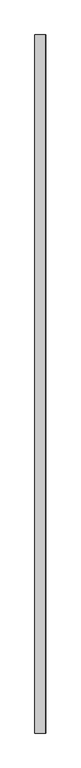
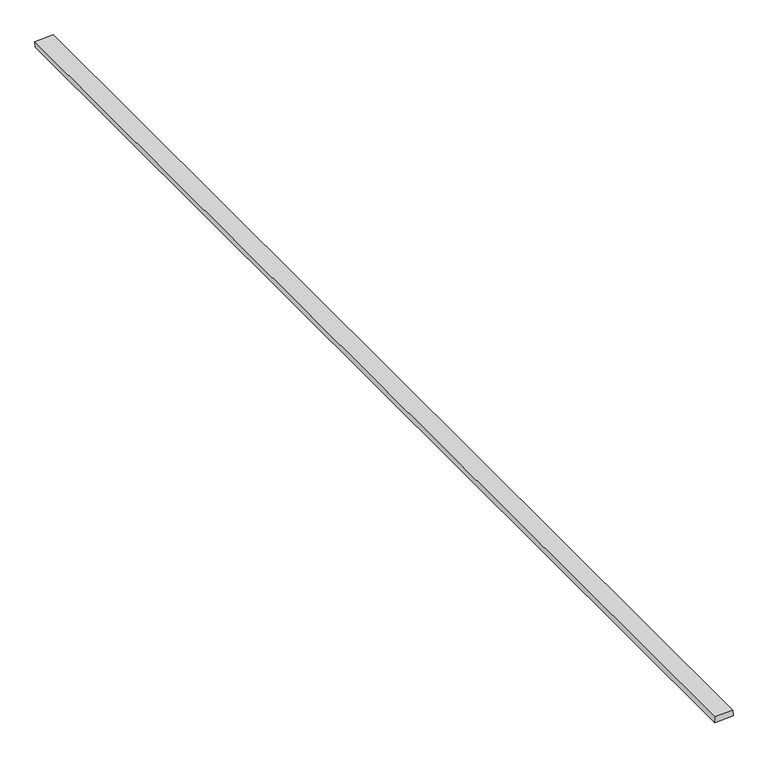
"""IFC4 building model written with IfcOpenShell, lengths in millimetres: proxy geometry, Inner panel:Inner panel:1:Inner panel:1 : Inner panel:Inner panel:300324:2:Inner panel:1:Inner panel:1 : Inner panel:Inner panel:300324:2 : Inner panel:Inner panel:1:Inner panel:1 : Inner panel:Inner panel:300324:300043:31 : Inner panel:Inner panel:1:Inner panel:1 : Inner panel:Inner panel:300324:2:Inner panel:1:Inner panel:1 : Inner panel:Inner panel:300324:2 : Inner panel:Inner panel:1:Inner panel:1 : Inner panel:Inner panel:300324:300043:308120."""

from ifc_helpers import new_model, si_unit, frame, origin, place, context, project, spatial, polyline, outline, extrude, source, transform, mapped, element, save


def generic_models_3c92ea3c(model_context):
    return source(origin(), model_context, "Body", "SweptSolid", [
        extrude(outline(polyline([(0.0, -75.8934963), (0.0, 0.0), (4876.8, 0.0), (4876.8, -75.8934963), (0.0, -75.8934963)])), frame((562974.8042403, -578718.116384, 4033.1905839), z_axis=(-0.04163054471215047, 0.0, 0.9991330730923532), x_axis=(0.0, 1.0, 0.0)), (0.0, 0.0, 1.0), 25.4),
    ])


if __name__ == "__main__":
    model = new_model("IFC4")
    model_context = context("Model", 3, world=origin())
    ifc_project = project(units=[si_unit("LENGTHUNIT", "METRE", prefix="MILLI")], contexts=[model_context])
    site = spatial("IfcSite", under=ifc_project)
    building = spatial("IfcBuilding", under=site)
    placement = place(None, origin())
    generic_models_shape = generic_models_3c92ea3c(model_context)
    element("IfcBuildingElementProxy", 1, Name="Inner panel:Inner panel:1:Inner panel:1 : Inner panel:Inner panel:300324:2:Inner panel:1:Inner panel:1 : Inner panel:Inner panel:300324:2 : Inner panel:Inner panel:1:Inner panel:1 : Inner panel:Inner panel:300324:300043:31 : Inner panel:Inner panel:1:Inner panel:1 : Inner panel:Inner panel:300324:2:Inner panel:1:Inner panel:1 : Inner panel:Inner panel:300324:2 : Inner panel:Inner panel:1:Inner panel:1 : Inner panel:Inner panel:300324:300043:308120", ObjectType="Inner panel:Inner panel:1:Inner panel:1 : Inner panel:Inner panel:300324:2:Inner panel:1:Inner panel:1 : Inner panel:Inner panel:300324:2 : Inner panel:Inner panel:1:Inner panel:1 : Inner panel:Inner panel:300324:300043:31 : Inner panel:Inner panel:1:Inner panel:1 : Inner panel:Inner panel:300324:2:Inner panel:1:Inner panel:1 : Inner panel:Inner panel:300324:2 : Inner panel:Inner panel:1:Inner panel:1 : Inner panel:Inner panel:300324:300043:308120", at=placement, inside=building, context=model_context, shape_type="MappedRepresentation", body=[
        mapped(generic_models_shape, transform((0.0, 0.0, 0.0), x_axis=(1.0, 0.0, 0.0), y_axis=(0.0, 1.0, 0.0), z_axis=(0.0, 0.0, 1.0))),
    ])
    save(model, "model.ifc")

# Revit data of these elements
# Type "Inner panel:Inner panel:1:Inner panel:1 : Inner panel:Inner panel:300324:2:Inner panel:1:Inner panel:1 : Inner panel:Inner panel:300324:2 : Inner panel:Inner panel:1:Inner panel:1 : Inner panel:Inner panel:300324:300043:31 : Inner panel:Inner panel:1:Inner panel:1 : Inner panel:Inner panel:300324:2:Inner panel:1:Inner panel:1 : Inner panel:Inner panel:300324:2 : Inner panel:Inner panel:1:Inner panel:1 : Inner panel:Inner panel:300324:300043:308120"
#   NameOverride = "Inner panel:Inner panel:1:Inner panel:1 : Inner panel:Inner panel:300324:2:Inner panel:1:Inner panel:1 : Inner panel:Inner panel:300324:2 : Inner panel:Inner panel:1:Inner panel:1 : Inner panel:Inner panel:300324:300043:308120"
#   ObjectTypeOverride = "Inner panel:1:Inner panel:1 : Inner panel:Inner panel:300324:2 : Inner panel:Inner panel:1:Inner panel:1 : Inner panel:Inner panel:300324:300043"
#   Reference = "Inner panel"
#   Tag = "308120"
# Element 1 (IfcBuildingElementProxy, "Inner panel:Inner panel:1:Inner panel:1 : Inner panel:Inner panel:300324:2:Inner panel:1:Inner panel:1 : Inner panel:Inner panel:300324:2 : Inner panel:Inner panel:1:Inner panel:1 : Inner panel:Inner panel:300324:300043:31 : Inner panel:Inner panel:1:Inner panel:1 : Inner panel:Inner panel:300324:2:Inner panel:1:Inner panel:1 : Inner panel:Inner panel:300324:2 : Inner panel:Inner panel:1:Inner panel:1 : Inner panel:Inner panel:300324:300043:308120")
#   Materials on its faces: "1\" THERMAL SPACER @ PURLIN"
# Materials
#   "1\" THERMAL SPACER @ PURLIN": class "Unassigned", colour RGB 205 188 106, transparency 0, Cost = 0
